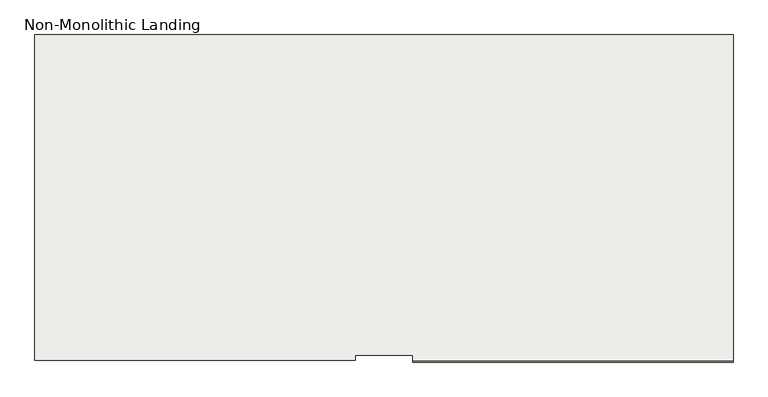
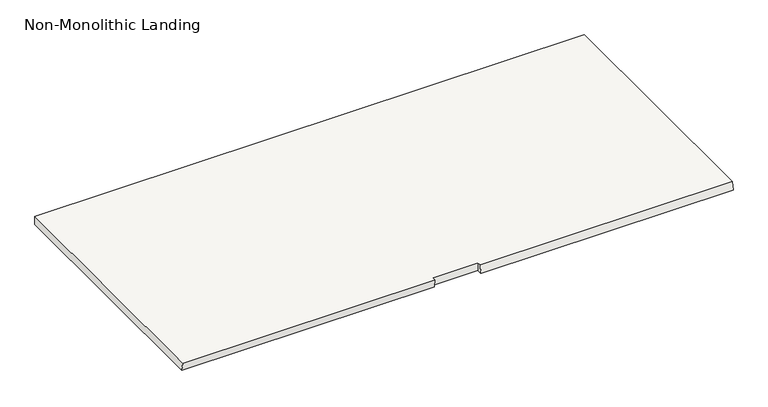
"""IFC4 building model written with IfcOpenShell, lengths in millimetres: slab geometry, Non-Monolithic Landing."""

from ifc_helpers import new_model, si_unit, origin, place, context, project, spatial, faceted_brep, source, transform, mapped, element, save


def non_monolithic_landing_893569eb(model_context):
    return source(origin(), model_context, "Body", "Brep", [
        faceted_brep([(-226.7120949, 7307.4781803, 11617.6470588), (-226.7120949, 7300.3948469, 11567.6470588), (1293.2879051, 7300.3948469, 11567.6470588), (1293.2879051, 7307.4781803, 11617.6470588), (-499.4393676, 7309.7509075, 11617.6470588), (-499.4393676, 7332.4781803, 11617.6470588), (-226.7120949, 7332.4781803, 11617.6470588), (1293.2879051, 7332.4781803, 11617.6470588), (1293.2879051, 8852.4781803, 11617.6470588), (-2019.4393676, 8852.4781803, 11617.6470588), (-2019.4393676, 7309.7509075, 11617.6470588), (-226.7120949, 7332.4781803, 11567.6470588), (-499.4393676, 7332.4781803, 11567.6470588), (-499.4393676, 7316.8342409, 11567.6470588), (-2019.4393676, 7316.8342409, 11567.6470588), (-2019.4393676, 8852.4781803, 11567.6470588), (1293.2879051, 8852.4781803, 11567.6470588), (1293.2879051, 7332.4781803, 11567.6470588)], [[[0, 1, 2, 3]], [[4, 5, 6, 0, 3, 7, 8, 9, 10]], [[11, 12, 13, 14, 15, 16, 17, 2, 1]], [[5, 4, 13, 12]], [[6, 5, 12, 11]], [[0, 6, 11, 1]], [[7, 3, 2, 17]], [[8, 7, 17, 16]], [[9, 8, 16, 15]], [[10, 9, 15, 14]], [[4, 10, 14, 13]]]),
    ])


if __name__ == "__main__":
    model = new_model("IFC4")
    model_context = context("Model", 3, world=origin())
    ifc_project = project(units=[si_unit("LENGTHUNIT", "METRE", prefix="MILLI")], contexts=[model_context])
    site = spatial("IfcSite", under=ifc_project)
    building = spatial("IfcBuilding", under=site)
    placement = place(None, origin())
    non_monolithic_landing_shape = non_monolithic_landing_893569eb(model_context)
    element("IfcSlab", 1, ObjectType="Non-Monolithic Landing", at=placement, inside=building, context=model_context, shape_type="MappedRepresentation", body=[
        mapped(non_monolithic_landing_shape, transform((0.0, 0.0, 0.0), x_axis=(1.0, 0.0, 0.0), y_axis=(0.0, 1.0, 0.0), z_axis=(0.0, 0.0, 1.0))),
    ])
    save(model, "model.ifc")
